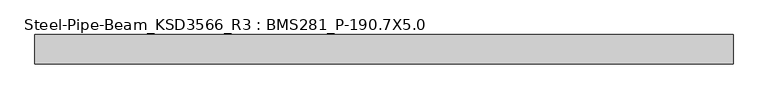
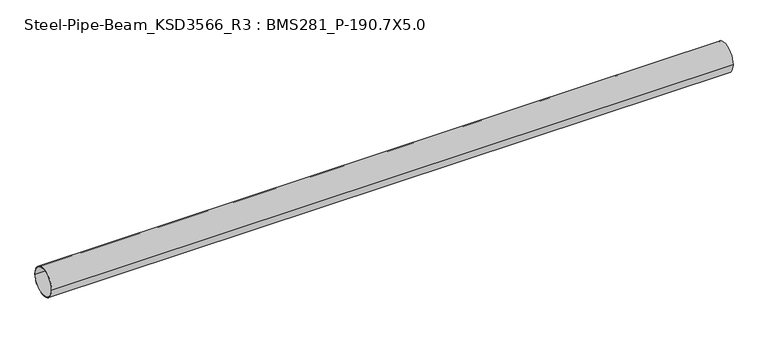
"""IFC4 building model written with IfcOpenShell, lengths in millimetres: member geometry, Steel-Pipe-Beam_KSD3566_R3 : BMS281_P-190.7X5.0."""

from ifc_helpers import new_model, si_unit, point, frame, origin, origin_2d, place, context, project, spatial, circle_curve, trimmed, segment, composite_curve, outline, extrude, source, transform, mapped, element, save


def steel_pipe_beam_ksd3566_r3_bms281_p_190_7x5_0_12fcad8a(model_context):
    return source(origin(), model_context, "Body", "SweptSolid", [
        extrude(outline(composite_curve([segment(trimmed(circle_curve(origin_2d(), 95.35), [point((-95.35, 0.0))], [point((95.35, 0.0))], False, "CARTESIAN"), True, "CONTINUOUS"), segment(trimmed(circle_curve(origin_2d(), 95.35), [point((95.35, 0.0))], [point((-95.35, 0.0))], False, "CARTESIAN"), True, "CONTINUOUS")], self_intersect=False), holes=[composite_curve([segment(trimmed(circle_curve(origin_2d(), 90.35), [point((90.35, 0.0))], [point((-90.35, 0.0))], True, "CARTESIAN"), True, "CONTINUOUS"), segment(trimmed(circle_curve(origin_2d(), 90.35), [point((-90.35, 0.0))], [point((90.35, 0.0))], True, "CARTESIAN"), True, "CONTINUOUS")], self_intersect=False)]), frame((-2227.6376817, 0.0, 0.0), z_axis=(1.0, 0.0, 0.0), x_axis=(0.0, 1.0, 0.0)), (0.0, 0.0, 1.0), 4533.0400738),
    ])


if __name__ == "__main__":
    model = new_model("IFC4")
    model_context = context("Model", 3, world=origin())
    ifc_project = project(units=[si_unit("LENGTHUNIT", "METRE", prefix="MILLI")], contexts=[model_context])
    site = spatial("IfcSite", under=ifc_project)
    building = spatial("IfcBuilding", under=site)
    placement = place(None, origin())
    steel_pipe_beam_ksd3566_r3_bms281_p_190_7x5_0_shape = steel_pipe_beam_ksd3566_r3_bms281_p_190_7x5_0_12fcad8a(model_context)
    element("IfcMember", 1, ObjectType="Steel-Pipe-Beam_KSD3566_R3 : BMS281_P-190.7X5.0", at=placement, inside=building, context=model_context, shape_type="MappedRepresentation", body=[
        mapped(steel_pipe_beam_ksd3566_r3_bms281_p_190_7x5_0_shape, transform((0.0, 0.0, 0.0), x_axis=(1.0, 0.0, 0.0), y_axis=(0.0, 1.0, 0.0), z_axis=(0.0, 0.0, 1.0))),
    ])
    save(model, "model.ifc")

# Revit data of these elements
# Type "Steel-Pipe-Beam_KSD3566_R3 : BMS281_P-190.7X5.0"
#   Keynote = "P-190.7X5.0"
#   SteelWeight = "Light"
#   t = 0.0050 m
#   Surface Area = 0.599102 m²/m
#   Section Area = 29.1697 cm²
#   Mass per Unit Length = 22.8982 kg/m
#   Length [instance default] = 1.5000 m
#   D = 0.1907 m
#   hec_material4 [instance default] = none
#   hec_material3 [instance default] = none
#   hec_material2 [instance default] = none
#   hec_material1 [instance default] = none
#   Structural Material [instance default] = Steel, 45-345
#   Assembly Code = ""
# Element 1 (IfcMember, "Steel-Pipe-Beam_KSD3566_R3 : BMS281_P-190.7X5.0")
#   Structural Material = none
# Materials
#   "Steel, 45-345": class "Metal", colour RGB 189 187 185, transparency 0, Description = "Steel 345 MPa", Cost = 0
